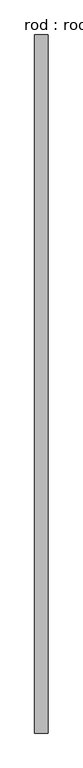
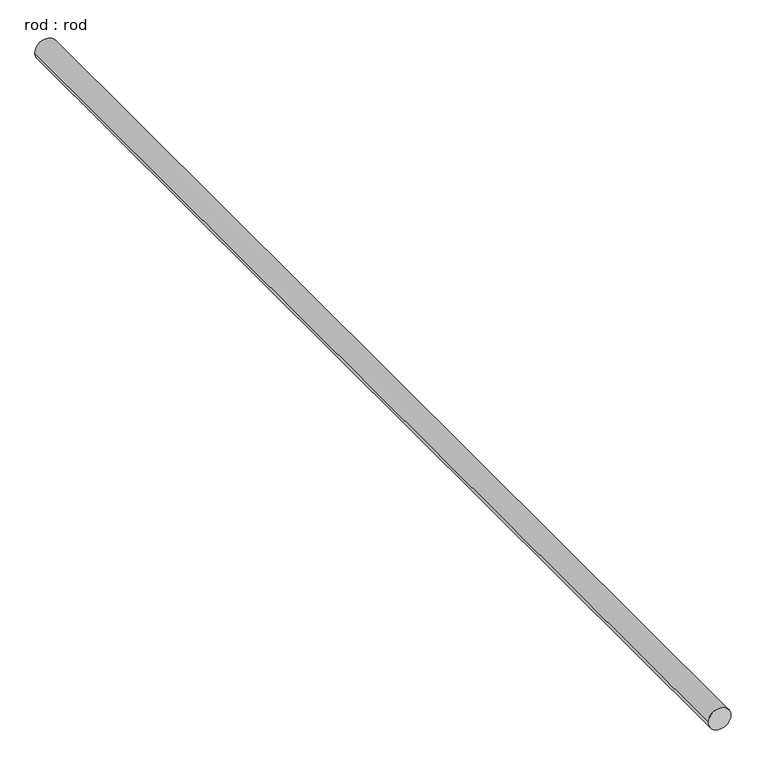
"""IFC4 building model written with IfcOpenShell, lengths in millimetres: proxy geometry, rod : rod."""

from ifc_helpers import new_model, si_unit, point, frame, frame_2d, origin, place, context, project, spatial, circle_curve, trimmed, segment, composite_curve, outline, extrude, source, transform, mapped, element, save


def rod_rod_e55882fe(model_context):
    return source(origin(), model_context, "Body", "SweptSolid", [
        extrude(outline(composite_curve([segment(trimmed(circle_curve(frame_2d((0.0108462, 0.0)), 200.0), [point((0.0108462, 200.0))], [point((0.0108462, -200.0))], False, "CARTESIAN"), True, "CONTINUOUS"), segment(trimmed(circle_curve(frame_2d((0.0108462, 0.0)), 200.0), [point((0.0108462, -200.0))], [point((0.0108462, 200.0))], False, "CARTESIAN"), True, "CONTINUOUS")], self_intersect=False)), frame((0.0, -6282.2713847, 0.0), z_axis=(0.0, 1.0, 0.0), x_axis=(0.0, 0.0, 1.0)), (0.0, 0.0, 1.0), 20750.0),
    ])


if __name__ == "__main__":
    model = new_model("IFC4")
    model_context = context("Model", 3, world=origin())
    ifc_project = project(units=[si_unit("LENGTHUNIT", "METRE", prefix="MILLI")], contexts=[model_context])
    site = spatial("IfcSite", under=ifc_project)
    building = spatial("IfcBuilding", under=site)
    placement = place(None, origin())
    rod_rod_shape = rod_rod_e55882fe(model_context)
    element("IfcBuildingElementProxy", 1, Name="rod : rod", ObjectType="rod : rod", at=placement, inside=building, context=model_context, shape_type="MappedRepresentation", body=[
        mapped(rod_rod_shape, transform((0.0, 0.0, 0.0), x_axis=(1.0, 0.0, 0.0), y_axis=(0.0, 1.0, 0.0), z_axis=(0.0, 0.0, 1.0))),
    ])
    save(model, "model.ifc")

# Revit data of these elements
# Type "rod : rod"
#   Default Elevation = 0
